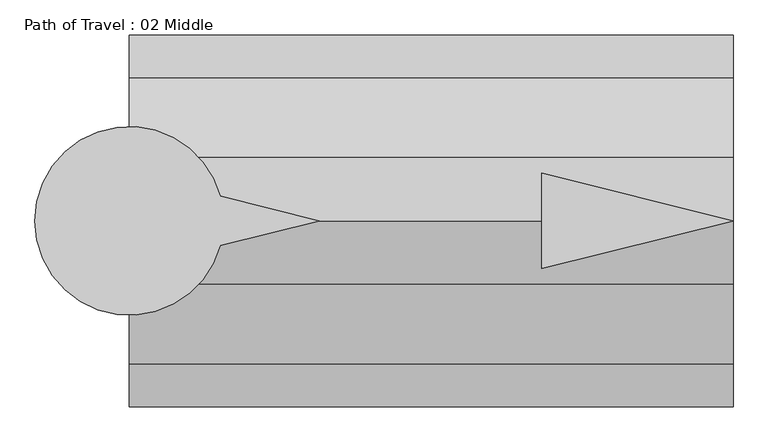
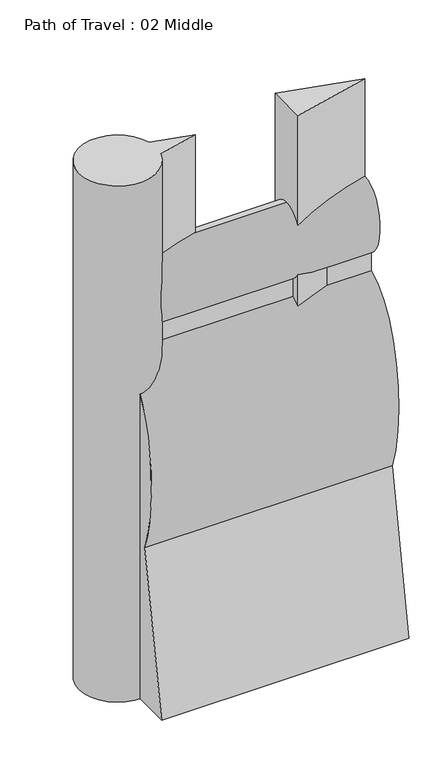
"""IFC4 building model written with IfcOpenShell, lengths in millimetres: proxy geometry, Path of Travel : 02 Middle."""

from ifc_helpers import new_model, si_unit, point, frame, frame_2d, origin, origin_with_axes, place, context, project, spatial, polyline, circle_curve, ellipse_curve, trimmed, segment, composite_curve, outline, extrude, source, transform, mapped, element, save
from ifc_brep_helpers import plane_surface, extruded_surface, advanced_brep


def path_of_travel_02_middle_0746a8d3(model_context):
    return source(origin(), model_context, "Body", "SolidModel", [
        advanced_brep(
        [(227.5554837, 0.0, 1727.2), (227.5554837, 42.9018657, 1436.6534209), (227.5554837, 42.9018657, 1363.4763406), (227.5554837, 184.1186263, 643.4144547), (227.5554837, 297.5699544, 0.0), (227.5554837, 145.6574193, 0.0), (227.5554837, 0.0, 584.2), (227.5554837, -145.6574193, 0.0), (227.5554837, -297.5699544, 0.0), (227.5554837, -184.1186263, 643.4144547), (227.5554837, -42.9018657, 1363.4763406), (227.5554837, -42.9018657, 1436.6534209), (1192.7554837, 0.0, 1727.2), (1192.7554837, -42.9018657, 1436.6534209), (1192.7554837, -42.9018657, 1363.4763406), (1192.7554837, -184.1186263, 643.4144547), (1192.7554837, -297.5699544, 0.0), (1192.7554837, -145.6574193, 0.0), (1192.7554837, 0.0, 584.2), (1192.7554837, 145.6574193, 0.0), (1192.7554837, 297.5699544, 0.0), (1192.7554837, 184.1186263, 643.4144547), (1192.7554837, 42.9018657, 1363.4763406), (1192.7554837, 42.9018657, 1436.6534209)],
        [
            (0, 1, ellipse_curve(frame((227.5554837, 0.0, 1574.8), z_axis=(-1.0, 0.0, 0.0), x_axis=(0.0, 0.0, 1.0)), 152.4, 101.6)),
            (1, 2),
            (2, 3, ellipse_curve(frame((227.5554837, 0.0, 914.4), z_axis=(-1.0, 0.0, 0.0), x_axis=(0.0, 0.0, -1.0)), 457.2, 228.6)),
            (3, 4),
            (4, 5),
            (5, 6),
            (6, 7),
            (7, 8),
            (8, 9),
            (9, 10, ellipse_curve(frame((227.5554837, 0.0, 914.4), z_axis=(-1.0, 0.0, 0.0), x_axis=(0.0, 0.0, -1.0)), 457.2, 228.6)),
            (10, 11),
            (11, 0, ellipse_curve(frame((227.5554837, 0.0, 1574.8), z_axis=(-1.0, 0.0, 0.0), x_axis=(0.0, 0.0, 1.0)), 152.4, 101.6)),
            (12, 13, ellipse_curve(frame((1192.7554837, 0.0, 1574.8), z_axis=(1.0, 0.0, 0.0), x_axis=(0.0, 0.0, 1.0)), 152.4, 101.6)),
            (13, 14),
            (14, 15, ellipse_curve(frame((1192.7554837, 0.0, 914.4), z_axis=(1.0, 0.0, 0.0), x_axis=(0.0, 0.0, -1.0)), 457.2, 228.6)),
            (15, 16),
            (16, 17),
            (17, 18),
            (18, 19),
            (19, 20),
            (20, 21),
            (21, 22, ellipse_curve(frame((1192.7554837, 0.0, 914.4), z_axis=(1.0, 0.0, 0.0), x_axis=(0.0, 0.0, -1.0)), 457.2, 228.6)),
            (22, 23),
            (23, 12, ellipse_curve(frame((1192.7554837, 0.0, 1574.8), z_axis=(1.0, 0.0, 0.0), x_axis=(0.0, 0.0, 1.0)), 152.4, 101.6)),
            (0, 12),
            (23, 1),
            (22, 2),
            (21, 3),
            (20, 4),
            (19, 5),
            (18, 6),
            (17, 7),
            (16, 8),
            (15, 9),
            (14, 10),
            (13, 11),
        ],
        [
            plane_surface(frame((227.5554837, 0.0, 0.0), z_axis=(-1.0, 0.0, 0.0), x_axis=(0.0, 0.0, 1.0))),
            plane_surface(frame((1192.7554837, 0.0, 0.0), z_axis=(1.0, 0.0, 0.0), x_axis=(0.0, 0.0, 1.0))),
            extruded_surface(trimmed(ellipse_curve(frame((1192.7554837, 0.0, 1574.8), z_axis=(-1.0, 0.0, 0.0), x_axis=(0.0, 0.0, 1.0)), 152.4, 101.6), [point((1192.7554837, 0.0, 1727.2))], [point((1192.7554837, 42.9018657, 1436.6534209))], True, "CARTESIAN"), (-965.2, 0.0, 0.0), 965.2),
            plane_surface(frame((227.5554837, 42.9018657, 1436.6534209), z_axis=(0.0, 1.0, 0.0), x_axis=(1.0, 0.0, 0.0))),
            extruded_surface(trimmed(ellipse_curve(frame((1192.7554837, 0.0, 914.4), z_axis=(-1.0, 0.0, 0.0), x_axis=(0.0, 0.0, -1.0)), 457.2, 228.6), [point((1192.7554837, 42.9018657, 1363.4763406))], [point((1192.7554837, 184.1186263, 643.4144547))], True, "CARTESIAN"), (-965.2, 0.0, 0.0), 965.2),
            plane_surface(frame((227.5554837, 184.1186263, 643.4144547), z_axis=(0.0, 0.9848077530122078, 0.1736481776669322), x_axis=(1.0, 0.0, 0.0))),
            plane_surface(frame((227.5554837, 297.5699544, 0.0), z_axis=(0.0, 0.0, -1.0), x_axis=(1.0, 0.0, 0.0))),
            plane_surface(frame((227.5554837, 145.6574193, 0.0), z_axis=(0.0, -0.9702957262760199, -0.2419218955995739), x_axis=(1.0, 0.0, 0.0))),
            plane_surface(frame((227.5554837, 0.0, 584.2), z_axis=(0.0, 0.9702957262759961, -0.24192189559966923), x_axis=(1.0, 0.0, 0.0))),
            plane_surface(frame((227.5554837, -145.6574193, 0.0), z_axis=(0.0, 0.0, -1.0), x_axis=(1.0, 0.0, 0.0))),
            plane_surface(frame((227.5554837, -297.5699544, 0.0), z_axis=(0.0, -0.984807753012208, 0.17364817766693066), x_axis=(1.0, 0.0, 0.0))),
            extruded_surface(trimmed(ellipse_curve(frame((1192.7554837, 0.0, 914.4), z_axis=(-1.0, 0.0, 0.0), x_axis=(0.0, 0.0, -1.0)), 457.2, 228.6), [point((1192.7554837, -184.1186263, 643.4144547))], [point((1192.7554837, -42.9018657, 1363.4763406))], True, "CARTESIAN"), (-965.2, 0.0, 0.0), 965.2),
            plane_surface(frame((227.5554837, -42.9018657, 1363.4763406), z_axis=(0.0, -1.0, 0.0), x_axis=(1.0, 0.0, 0.0))),
            extruded_surface(trimmed(ellipse_curve(frame((1192.7554837, 0.0, 1574.8), z_axis=(-1.0, 0.0, 0.0), x_axis=(0.0, 0.0, 1.0)), 152.4, 101.6), [point((1192.7554837, -42.9018657, 1436.6534209))], [point((1192.7554837, 0.0, 1727.2))], True, "CARTESIAN"), (-965.2, 0.0, 0.0), 965.2),
        ],
        [
            (0, [[1, 2, 3, 4, 5, 6, 7, 8, 9, 10, 11, 12]]),
            (1, [[13, 14, 15, 16, 17, 18, 19, 20, 21, 22, 23, 24]]),
            (2, [[-1, 25, -24, 26]]),
            (3, [[-2, -26, -23, 27]]),
            (4, [[-3, -27, -22, 28]]),
            (5, [[-4, -28, -21, 29]]),
            (6, [[-5, -29, -20, 30]]),
            (7, [[-6, -30, -19, 31]]),
            (8, [[-7, -31, -18, 32]]),
            (9, [[-8, -32, -17, 33]]),
            (10, [[-9, -33, -16, 34]]),
            (11, [[-10, -34, -15, 35]]),
            (12, [[-11, -35, -14, 36]]),
            (13, [[-12, -36, -13, -25]]),
        ],
    ),
        extrude(outline(polyline([(886.7503371, 76.2006338), (1192.7554837, 0.0), (886.7503371, -76.2006338), (886.7503371, 76.2006338)])), origin_with_axes(), (0.0, 0.0, 1.0), 2129.5973753),
        extrude(outline(composite_curve([segment(polyline([(372.7837828, 39.4440225), (531.182385, 0.0), (372.7837828, -39.4440225)]), True, "CONTINUOUS"), segment(trimmed(circle_curve(frame_2d((227.2200886, 0.0)), 150.8131956), [point((372.7837828, -39.4440225))], [point((372.7837828, 39.4440225))], False, "CARTESIAN"), True, "CONTINUOUS")], self_intersect=False)), origin_with_axes(), (0.0, 0.0, 1.0), 2129.5973753),
    ])


if __name__ == "__main__":
    model = new_model("IFC4")
    model_context = context("Model", 3, world=origin())
    ifc_project = project(units=[si_unit("LENGTHUNIT", "METRE", prefix="MILLI")], contexts=[model_context])
    site = spatial("IfcSite", under=ifc_project)
    building = spatial("IfcBuilding", under=site)
    placement = place(None, origin())
    path_of_travel_02_middle_shape = path_of_travel_02_middle_0746a8d3(model_context)
    element("IfcBuildingElementProxy", 1, Name="Path of Travel : 02 Middle", ObjectType="Path of Travel : 02 Middle", at=placement, inside=building, context=model_context, shape_type="MappedRepresentation", body=[
        mapped(path_of_travel_02_middle_shape, transform((0.0, 0.0, 0.0), x_axis=(1.0, 0.0, 0.0), y_axis=(0.0, 1.0, 0.0), z_axis=(0.0, 0.0, 1.0))),
    ])
    save(model, "model.ifc")

# Revit data of these elements
# Type "Path of Travel : 02 Middle"
#   Path of Egress [instance default] = 4' - 0"
#   built-in parameter 1001306 [instance default] = 4 (stored number, unit not read)
#   Dot at Start = no
#   Arrow in Middle = yes
#   Arrow at End = no
#   Egress Path = none
# Element 1 (IfcBuildingElementProxy, "Path of Travel : 02 Middle")
#   Path of Egress = 3' - 2"
#   built-in parameter 1001306 = 3.16667 (stored number, unit not read)
#   Materials on its faces: "Egress Path Solid", "solid"
# Materials
#   "Egress Path Solid": class "Unassigned", colour RGB 255 128 64, transparency 0.75, Comments = "Rendering appearance not upgraded "
#   "solid": class "Generic", colour RGB 120 120 120, transparency 0, Cost = 0
